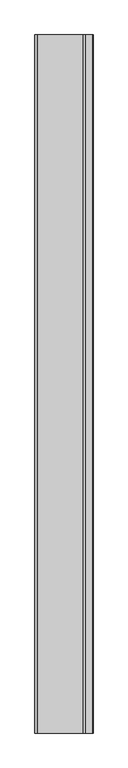
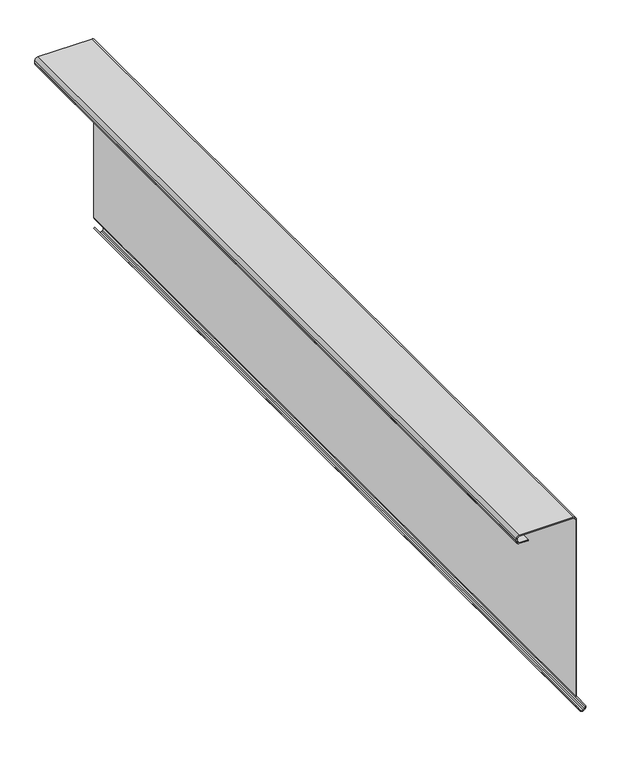
"""IFC4 building model written with IfcOpenShell, lengths in millimetres: proxy geometry, Flashing8:Flashing018:292359 : Flashing8:Flashing018:292359."""

from ifc_helpers import new_model, si_unit, point, frame, frame_2d, origin, place, context, project, spatial, polyline, circle_curve, trimmed, segment, composite_curve, outline, extrude, source, transform, mapped, element, save


def generic_models_8f9db25f(model_context):
    return source(origin(), model_context, "Body", "SweptSolid", [
        extrude(outline(composite_curve([segment(trimmed(circle_curve(frame_2d((43039.8127852, 22540.438897)), 5.08), [point((43035.7012799, 22543.4225063))], [point((43036.8907248, 22536.2834231))], True, "CARTESIAN"), True, "CONTINUOUS"), segment(polyline([(43036.8907248, 22536.2834231), (43051.477598, 22526.0261757), (43050.3271805, 22524.3901623), (43035.7403074, 22534.6474097)]), True, "CONTINUOUS"), segment(trimmed(circle_curve(frame_2d((43039.8127852, 22540.438897)), 7.08), [point((43035.7403074, 22534.6474097))], [point((43034.0825771, 22544.5971556))], False, "CARTESIAN"), True, "CONTINUOUS"), segment(polyline([(43034.0825771, 22544.5971556), (43035.3752562, 22546.3785071)]), True, "CONTINUOUS"), segment(trimmed(circle_curve(frame_2d((43041.1054643, 22542.2202485)), 7.08), [point((43035.3752562, 22546.3785071))], [point((43045.1570771, 22548.0263515))], False, "CARTESIAN"), True, "CONTINUOUS"), segment(polyline([(43045.1570771, 22548.0263515), (43075.4099277, 22526.9153177)]), True, "CONTINUOUS"), segment(trimmed(circle_curve(frame_2d((43077.1724938, 22529.4411366)), 3.08), [point((43075.4099277, 22526.9153177))], [point((43077.1724938, 22526.3611366))], True, "CARTESIAN"), True, "CONTINUOUS"), segment(polyline([(43077.1724938, 22526.3611366), (43524.4015043, 22526.3611366)]), True, "CONTINUOUS"), segment(trimmed(circle_curve(frame_2d((43524.4015043, 22519.2811366)), 7.08), [point((43524.4015043, 22526.3611366))], [point((43531.4815043, 22519.2811366))], False, "CARTESIAN"), True, "CONTINUOUS"), segment(polyline([(43531.4815043, 22519.2811366), (43531.4815043, 22389.9411366)]), True, "CONTINUOUS"), segment(trimmed(circle_curve(frame_2d((43524.4015043, 22389.9411366)), 7.08), [point((43531.4815043, 22389.9411366))], [point((43524.4015043, 22382.8611366))], False, "CARTESIAN"), True, "CONTINUOUS"), segment(polyline([(43524.4015043, 22382.8611366), (43517.995098, 22382.8611366)]), True, "CONTINUOUS"), segment(trimmed(circle_curve(frame_2d((43517.995098, 22389.9411366)), 7.08), [point((43517.995098, 22382.8611366))], [point((43510.915098, 22389.9411366))], False, "CARTESIAN"), True, "CONTINUOUS"), segment(polyline([(43510.915098, 22389.9411366), (43510.915098, 22411.2376015), (43512.915098, 22411.2376015), (43512.915098, 22389.9411366)]), True, "CONTINUOUS"), segment(trimmed(circle_curve(frame_2d((43517.995098, 22389.9411366)), 5.08), [point((43512.915098, 22389.9411366))], [point((43517.995098, 22384.8611366))], True, "CARTESIAN"), True, "CONTINUOUS"), segment(polyline([(43517.995098, 22384.8611366), (43524.4015043, 22384.8611366)]), True, "CONTINUOUS"), segment(trimmed(circle_curve(frame_2d((43524.4015043, 22389.9411366)), 5.08), [point((43524.4015043, 22384.8611366))], [point((43529.4815043, 22389.9411366))], True, "CARTESIAN"), True, "CONTINUOUS"), segment(polyline([(43529.4815043, 22389.9411366), (43529.4815043, 22519.2811366)]), True, "CONTINUOUS"), segment(trimmed(circle_curve(frame_2d((43524.4015043, 22519.2811366)), 5.08), [point((43529.4815043, 22519.2811366))], [point((43524.4015043, 22524.3611366))], True, "CARTESIAN"), True, "CONTINUOUS"), segment(polyline([(43524.4015043, 22524.3611366), (43077.1724938, 22524.3611366)]), True, "CONTINUOUS"), segment(trimmed(circle_curve(frame_2d((43077.1724938, 22529.4411366)), 5.08), [point((43077.1724938, 22524.3611366))], [point((43074.2654043, 22525.2751756))], False, "CARTESIAN"), True, "CONTINUOUS"), segment(polyline([(43074.2654043, 22525.2751756), (43044.0125537, 22546.3862094)]), True, "CONTINUOUS"), segment(trimmed(circle_curve(frame_2d((43041.1054643, 22542.2202485)), 5.08), [point((43044.0125537, 22546.3862094))], [point((43036.993959, 22545.2038578))], True, "CARTESIAN"), True, "CONTINUOUS"), segment(polyline([(43036.993959, 22545.2038578), (43035.7012799, 22543.4225063)]), True, "CONTINUOUS")], self_intersect=False)), frame((0.0, 8260.4833122, 0.0), z_axis=(0.0, 1.0, 0.0), x_axis=(0.0, 0.0, 1.0)), (0.0, 0.0, 1.0), 2000.0),
    ])


if __name__ == "__main__":
    model = new_model("IFC4")
    model_context = context("Model", 3, world=origin())
    ifc_project = project(units=[si_unit("LENGTHUNIT", "METRE", prefix="MILLI")], contexts=[model_context])
    site = spatial("IfcSite", under=ifc_project)
    building = spatial("IfcBuilding", under=site)
    placement = place(None, origin())
    generic_models_shape = generic_models_8f9db25f(model_context)
    element("IfcBuildingElementProxy", 1, Name="Flashing8:Flashing018:292359 : Flashing8:Flashing018:292359", ObjectType="Flashing8:Flashing018:292359 : Flashing8:Flashing018:292359", at=placement, inside=building, context=model_context, shape_type="MappedRepresentation", body=[
        mapped(generic_models_shape, transform((0.0, 0.0, 0.0), x_axis=(1.0, 0.0, 0.0), y_axis=(0.0, 1.0, 0.0), z_axis=(0.0, 0.0, 1.0))),
    ])
    save(model, "model.ifc")

# Revit data of these elements
# Type "Flashing8:Flashing018:292359 : Flashing8:Flashing018:292359"
#   NameOverride = "Flashing8:Flashing018:292359"
#   ObjectTypeOverride = "Flashing8:Flashing018"
#   Reference = "Flashing018"
#   Category = "Generic Models"
#   Tag = "292359"
# Element 1 (IfcBuildingElementProxy, "Flashing8:Flashing018:292359 : Flashing8:Flashing018:292359")
#   Materials on its faces: "HIGH EAVE FLASHING"
# Materials
#   "HIGH EAVE FLASHING": class "Unassigned", colour RGB 128 128 128, transparency 0, Cost = 0
